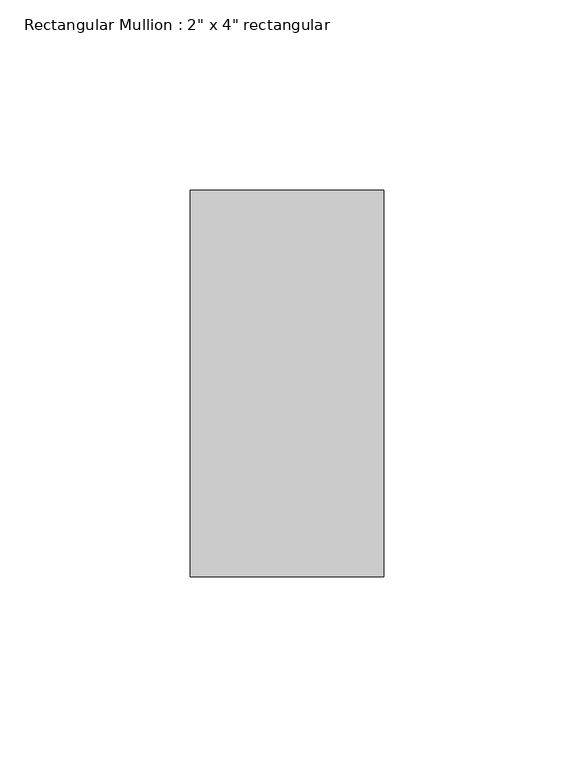
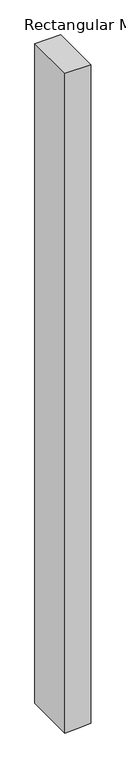
"""IFC4 building model written with IfcOpenShell, lengths in millimetres: member geometry."""

from ifc_helpers import new_model, si_unit, frame, origin, place, context, project, spatial, polyline, outline, extrude, source, transform, mapped, element, save


def member_202f567b(model_context):
    return source(origin(), model_context, "Body", "SweptSolid", [
        extrude(outline(polyline([(0.0, 25.4), (0.0, -25.4), (-1365.0533326, -25.4), (-1364.0831173, -2.1148317), (-1362.936666, 25.4), (0.0, 25.4)])), frame((0.0, -50.8, 0.0), z_axis=(0.0, 1.0, 0.0), x_axis=(0.0, 0.0, 1.0)), (0.0, 0.0, 1.0), 101.6),
    ])


if __name__ == "__main__":
    model = new_model("IFC4")
    model_context = context("Model", 3, world=origin())
    ifc_project = project(units=[si_unit("LENGTHUNIT", "METRE", prefix="MILLI")], contexts=[model_context])
    site = spatial("IfcSite", under=ifc_project)
    building = spatial("IfcBuilding", under=site)
    placement = place(None, origin())
    member_shape = member_202f567b(model_context)
    element("IfcMember", 1, ObjectType="Rectangular Mullion : 2\" x 4\" rectangular", at=placement, inside=building, context=model_context, shape_type="MappedRepresentation", body=[
        mapped(member_shape, transform((0.0, 0.0, 0.0), x_axis=(1.0, 0.0, 0.0), y_axis=(0.0, 1.0, 0.0), z_axis=(0.0, 0.0, 1.0))),
    ])
    save(model, "model.ifc")

# Revit data of these elements
# Type "Rectangular Mullion : 2\" x 4\" rectangular"
#   built-in parameter 1007304 = 0.333333 (stored number, unit not read)
#   built-in parameter 1007301 = 0.0833333 (stored number, unit not read)
#   built-in parameter 1007300 = 0.0833333 (stored number, unit not read)
# Element 1 (IfcMember, "Rectangular Mullion : 2\" x 4\" rectangular")
#   Materials on its faces: "PAINTED STEEL C CHANNEL"
# Materials
#   "PAINTED STEEL C CHANNEL": class "Generic", colour RGB 88 62 61, transparency 0, Cost = 0
